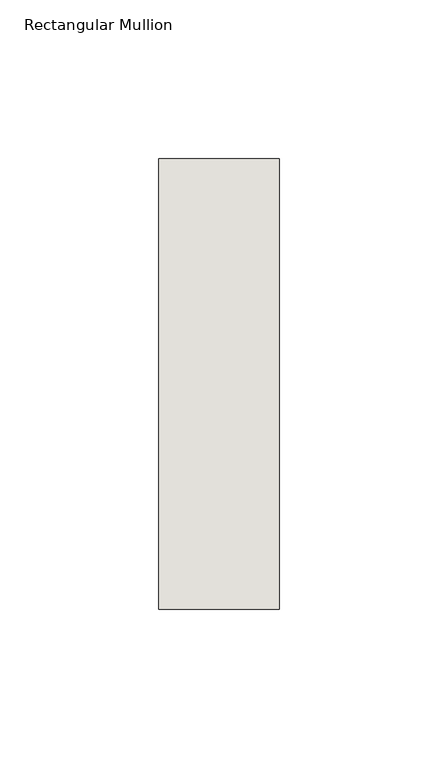
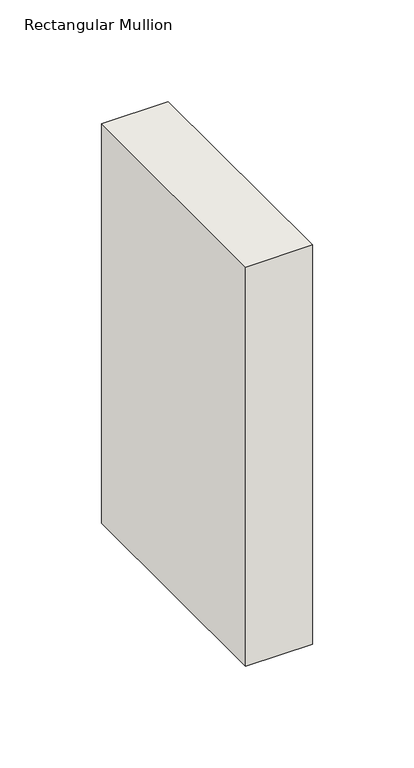
"""IFC4 building model written with IfcOpenShell, lengths in millimetres: wall geometry, Rectangular Mullion : NLRS_21_CWM_hsb-regel 38x142_gen_rsf."""

import ifcopenshell
import ifcopenshell.guid

model = None  # the IFC model being written
_history = None  # IfcOwnerHistory: only IFC2X3 demands one
_inside = {}  # id of a spatial element -> (the spatial element, [elements in it])
_under = {}  # id of a project, library or spatial element -> (it, [spatial elements below it])
_declared = {}  # id of a project -> (the project, [libraries it declares])
_typed = {}  # id of a type object -> (the type object, [elements of that type])
_made_of = {}  # id of a material, layer set ... -> (it, [elements and type objects made of it])


def new_model(schema):
    """Start an empty IFC model of exactly this schema.

    Asked for "IFC4X3", IfcOpenShell would pick the latest addendum, in which some entities
    have other attributes; the version numbers below select the first issue.
    IFC2X3 requires an IfcOwnerHistory on every rooted entity: one is made here for all.
    """
    global model, _history
    if schema == "IFC4X3":
        model = ifcopenshell.file(schema_version=(4, 3, 0, 0))
    else:
        model = ifcopenshell.file(schema=schema)
    _inside.clear()
    _under.clear()
    _declared.clear()
    _typed.clear()
    _made_of.clear()
    _history = None
    if model.schema == "IFC2X3":
        org = make("IfcOrganization", Name="unknown")
        user = make(
            "IfcPersonAndOrganization",
            ThePerson=make("IfcPerson", FamilyName="unknown"),
            TheOrganization=org,
        )
        app = make(
            "IfcApplication",
            ApplicationDeveloper=org,
            Version="unknown",
            ApplicationFullName="unknown",
            ApplicationIdentifier="unknown",
        )
        _history = make(
            "IfcOwnerHistory",
            OwningUser=user,
            OwningApplication=app,
            ChangeAction="ADDED",
            CreationDate=0,
        )
    return model


def make(cls, **values):
    """One entity of the class cls with the attributes given. An attribute that is None is left unset."""
    return model.create_entity(
        cls, **{name: value for name, value in values.items() if value is not None}
    )


def rooted(cls, **values):
    """An entity with a GlobalId (a new one), such as an element, a storey or a relation."""
    return make(cls, GlobalId=ifcopenshell.guid.new(), OwnerHistory=_history, **values)


def si_unit(unit_type, name, prefix=None):
    """IfcSIUnit, for example si_unit("LENGTHUNIT", "METRE", prefix="MILLI")."""
    return make("IfcSIUnit", UnitType=unit_type, Prefix=prefix, Name=name)


def assignment(units):
    """IfcUnitAssignment: the units of a project."""
    return None if units is None else make("IfcUnitAssignment", Units=units)


def point(xyz):
    """IfcCartesianPoint."""
    return None if xyz is None else make("IfcCartesianPoint", Coordinates=xyz)


def direction(xyz):
    """IfcDirection."""
    return None if xyz is None else make("IfcDirection", DirectionRatios=xyz)


def frame(location, z_axis=None, x_axis=None):
    """IfcAxis2Placement3D, a coordinate frame: its origin and axes. An axis left out is left unset."""
    return make(
        "IfcAxis2Placement3D",
        Location=point(location),
        Axis=direction(z_axis),
        RefDirection=direction(x_axis),
    )


def origin():
    """The frame at (0, 0, 0) with its axes left unset."""
    return frame((0.0, 0.0, 0.0))


def place(relative_to, where):
    """IfcLocalPlacement: puts the frame where relative to a parent placement (None: the world)."""
    return make(
        "IfcLocalPlacement", PlacementRelTo=relative_to, RelativePlacement=where
    )


def context(
    kind, dimensions, precision=None, world=None, true_north=None, identifier=None
):
    """IfcGeometricRepresentationContext, for example the 3D "Model" context."""
    return make(
        "IfcGeometricRepresentationContext",
        ContextIdentifier=identifier,
        ContextType=kind,
        CoordinateSpaceDimension=dimensions,
        Precision=precision,
        WorldCoordinateSystem=world,
        TrueNorth=true_north,
    )


def project(units=None, contexts=None):
    """IfcProject with its units and contexts."""
    return rooted(
        "IfcProject",
        Name="project",
        RepresentationContexts=contexts,
        UnitsInContext=assignment(units),
    )


def spatial(cls, under=None, at=None, **own):
    """A site, building, storey or space (cls), placed at a placement, below another one or the project."""
    s = rooted(cls, ObjectPlacement=at, **own)
    if under is not None:
        _under.setdefault(under.id(), (under, []))[1].append(s)
    return s


def polyline(points):
    """IfcPolyline through the points."""
    return make("IfcPolyline", Points=[point(p) for p in points])


def outline(outer, holes=None, kind="AREA"):
    """IfcArbitraryClosedProfileDef: a profile drawn as a closed curve; with holes, ...WithVoids."""
    if holes is None:
        return make("IfcArbitraryClosedProfileDef", ProfileType=kind, OuterCurve=outer)
    return make(
        "IfcArbitraryProfileDefWithVoids",
        ProfileType=kind,
        OuterCurve=outer,
        InnerCurves=holes,
    )


def extrude(swept, where, along, depth):
    """IfcExtrudedAreaSolid: the profile swept, set in the frame where, extruded along a direction by depth."""
    return make(
        "IfcExtrudedAreaSolid",
        SweptArea=swept,
        Position=where,
        ExtrudedDirection=direction(along),
        Depth=depth,
    )


def shape(context_of_items, identifier, shape_type, items):
    """IfcShapeRepresentation: the items that make up one representation, for example the "Body"."""
    return make(
        "IfcShapeRepresentation",
        ContextOfItems=context_of_items,
        RepresentationIdentifier=identifier,
        RepresentationType=shape_type,
        Items=items,
    )


def source(mapping_origin, context_of_items, identifier, shape_type, items):
    """IfcRepresentationMap: a shape defined once, which mapped items show again and again."""
    return make(
        "IfcRepresentationMap",
        MappingOrigin=mapping_origin,
        MappedRepresentation=shape(context_of_items, identifier, shape_type, items),
    )


def transform(
    local_origin,
    x_axis=None,
    y_axis=None,
    z_axis=None,
    scale=None,
    scale2=None,
    scale3=None,
    uniform=True,
):
    """IfcCartesianTransformationOperator3D, or its non-uniform kind. x_axis, y_axis, z_axis: its Axis1, 2, 3."""
    if uniform:
        return make(
            "IfcCartesianTransformationOperator3D",
            Axis1=direction(x_axis),
            Axis2=direction(y_axis),
            LocalOrigin=point(local_origin),
            Scale=scale,
            Axis3=direction(z_axis),
        )
    return make(
        "IfcCartesianTransformationOperator3DnonUniform",
        Axis1=direction(x_axis),
        Axis2=direction(y_axis),
        LocalOrigin=point(local_origin),
        Scale=scale,
        Axis3=direction(z_axis),
        Scale2=scale2,
        Scale3=scale3,
    )


def mapped(mapping_source, mapping_target):
    """IfcMappedItem: shows the shape of a source again, moved by a transform."""
    return make(
        "IfcMappedItem", MappingSource=mapping_source, MappingTarget=mapping_target
    )


def made_of(thing, what):
    """Note that an element or type object is made of a material, layer set ...; save() writes the relation."""
    if what is not None:
        _made_of.setdefault(what.id(), (what, []))[1].append(thing)
    return thing


def element(
    cls,
    number,
    at=None,
    inside=None,
    cuts=None,
    type_object=None,
    material=None,
    context=None,
    identifier="Body",
    shape_type=None,
    held_by="IfcProductDefinitionShape",
    body=None,
    shapes=None,
    **own,
):
    """One element of the class cls, such as IfcWall. Its Tag is "e" and its number.

    at: its placement. inside: the storey or other place that contains it. cuts: it is an
    opening in that element (IfcRelVoidsElement). A single representation is given by context,
    identifier, shape_type and body (its items); several are given by shapes. held_by: the class
    of the entity that holds the representations. save() writes the other relations.
    """
    e = rooted(cls, Tag="e%d" % number, ObjectPlacement=at, **own)
    if body is not None:
        shapes = [shape(context, identifier, shape_type, body)]
    if shapes is not None:
        e.Representation = make(held_by, Representations=shapes)
    if inside is not None:
        _inside.setdefault(inside.id(), (inside, []))[1].append(e)
    if cuts is not None:
        rooted(
            "IfcRelVoidsElement", RelatingBuildingElement=cuts, RelatedOpeningElement=e
        )
    if type_object is not None:
        _typed.setdefault(type_object.id(), (type_object, []))[1].append(e)
    return made_of(e, material)


def aggregate(whole, parts):
    """IfcRelAggregates: a whole, such as a stair, and the parts it consists of."""
    return rooted("IfcRelAggregates", RelatingObject=whole, RelatedObjects=parts)


def save(model, path):
    """Write the relations noted so far, then the file.

    IfcRelAggregates (storeys below a building ...), IfcRelContainedInSpatialStructure (elements
    in a storey), IfcRelDefinesByType, IfcRelAssociatesMaterial and IfcRelDeclares: one each for
    every whole, place, type object, material and project.
    """
    for whole, parts in _under.values():
        aggregate(whole, parts)
    for where, things in _inside.values():
        rooted(
            "IfcRelContainedInSpatialStructure",
            RelatedElements=things,
            RelatingStructure=where,
        )
    for kind, things in _typed.values():
        rooted("IfcRelDefinesByType", RelatedObjects=things, RelatingType=kind)
    for what, things in _made_of.values():
        rooted("IfcRelAssociatesMaterial", RelatedObjects=things, RelatingMaterial=what)
    for by, libraries in _declared.values():
        rooted("IfcRelDeclares", RelatingContext=by, RelatedDefinitions=libraries)
    model.write(path)


def rectangular_mullion_ad7c5b17(model_context):
    return source(origin(), model_context, "Body", "SweptSolid", [
        extrude(outline(polyline([(-38.0, -71.0), (-38.0, 71.0), (0.0, 71.0), (0.0, -71.0), (-38.0, -71.0)])), frame((0.0, 0.0, -239.8441061), z_axis=(0.0, 0.0, 1.0), x_axis=(1.0, 0.0, 0.0)), (0.0, 0.0, 1.0), 239.8441061),
    ])


if __name__ == "__main__":
    model = new_model("IFC4")
    model_context = context("Model", 3, world=origin())
    ifc_project = project(units=[si_unit("LENGTHUNIT", "METRE", prefix="MILLI")], contexts=[model_context])
    site = spatial("IfcSite", under=ifc_project)
    building = spatial("IfcBuilding", under=site)
    placement = place(None, origin())
    rectangular_mullion_shape = rectangular_mullion_ad7c5b17(model_context)
    element("IfcWall", 1, ObjectType="Rectangular Mullion : NLRS_21_CWM_hsb-regel 38x142_gen_rsf", at=placement, inside=building, context=model_context, shape_type="MappedRepresentation", body=[
        mapped(rectangular_mullion_shape, transform((0.0, 0.0, 0.0), x_axis=(1.0, 0.0, 0.0), y_axis=(0.0, 1.0, 0.0), z_axis=(0.0, 0.0, 1.0))),
    ])
    save(model, "model.ifc")

# Revit data of these elements
# Type "Rectangular Mullion : NLRS_21_CWM_hsb-regel 38x142_gen_rsf"
#   Type IfcGUID = "07M7mRoiH1CR8m_RSKIwpF"
#   Assembly Code = "21.10"
#   IfcExportAs = "IfcWall"
#   built-in parameter 1007322 = 0.465879 (stored number, unit not read)
#   built-in parameter 1007321 = 0.062336 (stored number, unit not read)
#   built-in parameter 1007320 = 0.062336 (stored number, unit not read)
# Element 1 (IfcWall, "Rectangular Mullion : NLRS_21_CWM_hsb-regel 38x142_gen_rsf")
#   Materials on its faces: "NLRS_i2_hout naaldhout vuren_gen_rsf"
# Materials
#   "NLRS_i2_hout naaldhout vuren_gen_rsf": class "I - Hout", colour RGB 234 199 147, transparency 0, Keynote = "i2", Manufacturer = "Revit Standards Foundation", URL = "www.revitstandards.org", Description = "hout vuren", Cost = 0
